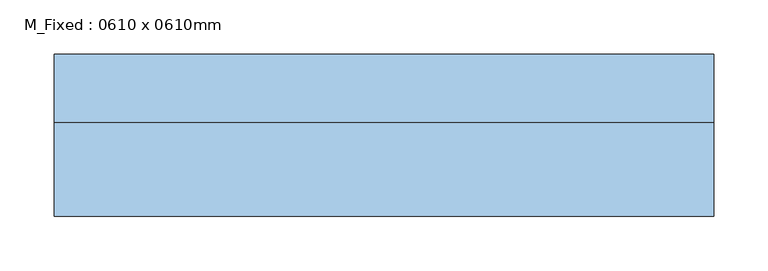
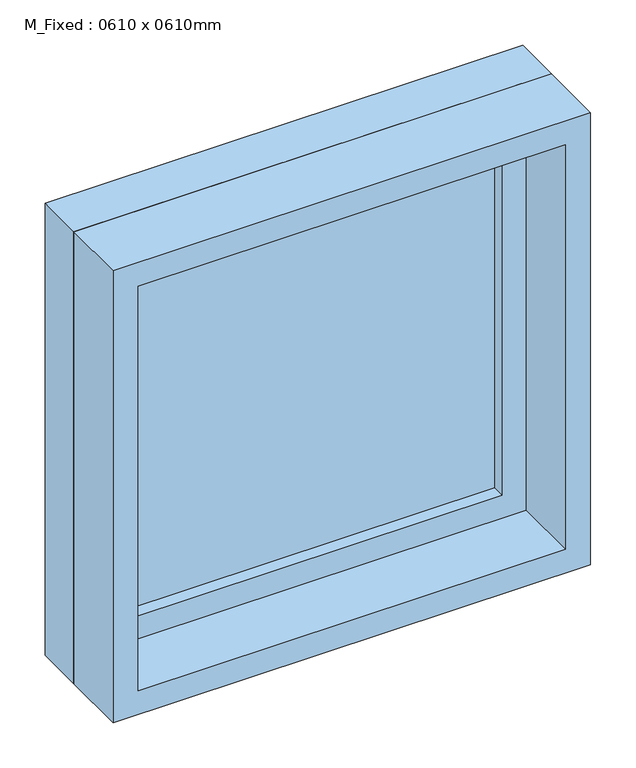
"""IFC4 building model written with IfcOpenShell, lengths in millimetres: window geometry, M_Fixed : 0610 x 0610mm."""

import ifcopenshell
import ifcopenshell.guid

model = None  # the IFC model being written
_history = None  # IfcOwnerHistory: only IFC2X3 demands one
_inside = {}  # id of a spatial element -> (the spatial element, [elements in it])
_under = {}  # id of a project, library or spatial element -> (it, [spatial elements below it])
_declared = {}  # id of a project -> (the project, [libraries it declares])
_typed = {}  # id of a type object -> (the type object, [elements of that type])
_made_of = {}  # id of a material, layer set ... -> (it, [elements and type objects made of it])


def new_model(schema):
    """Start an empty IFC model of exactly this schema.

    Asked for "IFC4X3", IfcOpenShell would pick the latest addendum, in which some entities
    have other attributes; the version numbers below select the first issue.
    IFC2X3 requires an IfcOwnerHistory on every rooted entity: one is made here for all.
    """
    global model, _history
    if schema == "IFC4X3":
        model = ifcopenshell.file(schema_version=(4, 3, 0, 0))
    else:
        model = ifcopenshell.file(schema=schema)
    _inside.clear()
    _under.clear()
    _declared.clear()
    _typed.clear()
    _made_of.clear()
    _history = None
    if model.schema == "IFC2X3":
        org = make("IfcOrganization", Name="unknown")
        user = make(
            "IfcPersonAndOrganization",
            ThePerson=make("IfcPerson", FamilyName="unknown"),
            TheOrganization=org,
        )
        app = make(
            "IfcApplication",
            ApplicationDeveloper=org,
            Version="unknown",
            ApplicationFullName="unknown",
            ApplicationIdentifier="unknown",
        )
        _history = make(
            "IfcOwnerHistory",
            OwningUser=user,
            OwningApplication=app,
            ChangeAction="ADDED",
            CreationDate=0,
        )
    return model


def make(cls, **values):
    """One entity of the class cls with the attributes given. An attribute that is None is left unset."""
    return model.create_entity(
        cls, **{name: value for name, value in values.items() if value is not None}
    )


def rooted(cls, **values):
    """An entity with a GlobalId (a new one), such as an element, a storey or a relation."""
    return make(cls, GlobalId=ifcopenshell.guid.new(), OwnerHistory=_history, **values)


def si_unit(unit_type, name, prefix=None):
    """IfcSIUnit, for example si_unit("LENGTHUNIT", "METRE", prefix="MILLI")."""
    return make("IfcSIUnit", UnitType=unit_type, Prefix=prefix, Name=name)


def assignment(units):
    """IfcUnitAssignment: the units of a project."""
    return None if units is None else make("IfcUnitAssignment", Units=units)


def point(xyz):
    """IfcCartesianPoint."""
    return None if xyz is None else make("IfcCartesianPoint", Coordinates=xyz)


def direction(xyz):
    """IfcDirection."""
    return None if xyz is None else make("IfcDirection", DirectionRatios=xyz)


def frame(location, z_axis=None, x_axis=None):
    """IfcAxis2Placement3D, a coordinate frame: its origin and axes. An axis left out is left unset."""
    return make(
        "IfcAxis2Placement3D",
        Location=point(location),
        Axis=direction(z_axis),
        RefDirection=direction(x_axis),
    )


def origin():
    """The frame at (0, 0, 0) with its axes left unset."""
    return frame((0.0, 0.0, 0.0))


def place(relative_to, where):
    """IfcLocalPlacement: puts the frame where relative to a parent placement (None: the world)."""
    return make(
        "IfcLocalPlacement", PlacementRelTo=relative_to, RelativePlacement=where
    )


def context(
    kind, dimensions, precision=None, world=None, true_north=None, identifier=None
):
    """IfcGeometricRepresentationContext, for example the 3D "Model" context."""
    return make(
        "IfcGeometricRepresentationContext",
        ContextIdentifier=identifier,
        ContextType=kind,
        CoordinateSpaceDimension=dimensions,
        Precision=precision,
        WorldCoordinateSystem=world,
        TrueNorth=true_north,
    )


def project(units=None, contexts=None):
    """IfcProject with its units and contexts."""
    return rooted(
        "IfcProject",
        Name="project",
        RepresentationContexts=contexts,
        UnitsInContext=assignment(units),
    )


def spatial(cls, under=None, at=None, **own):
    """A site, building, storey or space (cls), placed at a placement, below another one or the project."""
    s = rooted(cls, ObjectPlacement=at, **own)
    if under is not None:
        _under.setdefault(under.id(), (under, []))[1].append(s)
    return s


def polyline(points):
    """IfcPolyline through the points."""
    return make("IfcPolyline", Points=[point(p) for p in points])


def outline(outer, holes=None, kind="AREA"):
    """IfcArbitraryClosedProfileDef: a profile drawn as a closed curve; with holes, ...WithVoids."""
    if holes is None:
        return make("IfcArbitraryClosedProfileDef", ProfileType=kind, OuterCurve=outer)
    return make(
        "IfcArbitraryProfileDefWithVoids",
        ProfileType=kind,
        OuterCurve=outer,
        InnerCurves=holes,
    )


def extrude(swept, where, along, depth):
    """IfcExtrudedAreaSolid: the profile swept, set in the frame where, extruded along a direction by depth."""
    return make(
        "IfcExtrudedAreaSolid",
        SweptArea=swept,
        Position=where,
        ExtrudedDirection=direction(along),
        Depth=depth,
    )


def shape(context_of_items, identifier, shape_type, items):
    """IfcShapeRepresentation: the items that make up one representation, for example the "Body"."""
    return make(
        "IfcShapeRepresentation",
        ContextOfItems=context_of_items,
        RepresentationIdentifier=identifier,
        RepresentationType=shape_type,
        Items=items,
    )


def source(mapping_origin, context_of_items, identifier, shape_type, items):
    """IfcRepresentationMap: a shape defined once, which mapped items show again and again."""
    return make(
        "IfcRepresentationMap",
        MappingOrigin=mapping_origin,
        MappedRepresentation=shape(context_of_items, identifier, shape_type, items),
    )


def transform(
    local_origin,
    x_axis=None,
    y_axis=None,
    z_axis=None,
    scale=None,
    scale2=None,
    scale3=None,
    uniform=True,
):
    """IfcCartesianTransformationOperator3D, or its non-uniform kind. x_axis, y_axis, z_axis: its Axis1, 2, 3."""
    if uniform:
        return make(
            "IfcCartesianTransformationOperator3D",
            Axis1=direction(x_axis),
            Axis2=direction(y_axis),
            LocalOrigin=point(local_origin),
            Scale=scale,
            Axis3=direction(z_axis),
        )
    return make(
        "IfcCartesianTransformationOperator3DnonUniform",
        Axis1=direction(x_axis),
        Axis2=direction(y_axis),
        LocalOrigin=point(local_origin),
        Scale=scale,
        Axis3=direction(z_axis),
        Scale2=scale2,
        Scale3=scale3,
    )


def mapped(mapping_source, mapping_target):
    """IfcMappedItem: shows the shape of a source again, moved by a transform."""
    return make(
        "IfcMappedItem", MappingSource=mapping_source, MappingTarget=mapping_target
    )


def made_of(thing, what):
    """Note that an element or type object is made of a material, layer set ...; save() writes the relation."""
    if what is not None:
        _made_of.setdefault(what.id(), (what, []))[1].append(thing)
    return thing


def element(
    cls,
    number,
    at=None,
    inside=None,
    cuts=None,
    type_object=None,
    material=None,
    context=None,
    identifier="Body",
    shape_type=None,
    held_by="IfcProductDefinitionShape",
    body=None,
    shapes=None,
    **own,
):
    """One element of the class cls, such as IfcWall. Its Tag is "e" and its number.

    at: its placement. inside: the storey or other place that contains it. cuts: it is an
    opening in that element (IfcRelVoidsElement). A single representation is given by context,
    identifier, shape_type and body (its items); several are given by shapes. held_by: the class
    of the entity that holds the representations. save() writes the other relations.
    """
    e = rooted(cls, Tag="e%d" % number, ObjectPlacement=at, **own)
    if body is not None:
        shapes = [shape(context, identifier, shape_type, body)]
    if shapes is not None:
        e.Representation = make(held_by, Representations=shapes)
    if inside is not None:
        _inside.setdefault(inside.id(), (inside, []))[1].append(e)
    if cuts is not None:
        rooted(
            "IfcRelVoidsElement", RelatingBuildingElement=cuts, RelatedOpeningElement=e
        )
    if type_object is not None:
        _typed.setdefault(type_object.id(), (type_object, []))[1].append(e)
    return made_of(e, material)


def aggregate(whole, parts):
    """IfcRelAggregates: a whole, such as a stair, and the parts it consists of."""
    return rooted("IfcRelAggregates", RelatingObject=whole, RelatedObjects=parts)


def save(model, path):
    """Write the relations noted so far, then the file.

    IfcRelAggregates (storeys below a building ...), IfcRelContainedInSpatialStructure (elements
    in a storey), IfcRelDefinesByType, IfcRelAssociatesMaterial and IfcRelDeclares: one each for
    every whole, place, type object, material and project.
    """
    for whole, parts in _under.values():
        aggregate(whole, parts)
    for where, things in _inside.values():
        rooted(
            "IfcRelContainedInSpatialStructure",
            RelatedElements=things,
            RelatingStructure=where,
        )
    for kind, things in _typed.values():
        rooted("IfcRelDefinesByType", RelatedObjects=things, RelatingType=kind)
    for what, things in _made_of.values():
        rooted("IfcRelAssociatesMaterial", RelatedObjects=things, RelatingMaterial=what)
    for by, libraries in _declared.values():
        rooted("IfcRelDeclares", RelatingContext=by, RelatedDefinitions=libraries)
    model.write(path)


def m_fixed_0610_x_0610mm_d1ac9692(model_context):
    return source(origin(), model_context, "Body", "SweptSolid", [
        extrude(outline(polyline([(-242.0, 53.0), (242.0, 53.0), (242.0, 41.0), (-242.0, 41.0), (-242.0, 53.0)])), frame((0.0, 0.0, 978.0), z_axis=(0.0, 0.0, 1.0), x_axis=(1.0, 0.0, 0.0)), (0.0, 0.0, 1.0), 484.0),
        extrude(outline(polyline([(1506.0, -286.0), (934.0, -286.0), (934.0, 286.0), (1506.0, 286.0), (1506.0, -286.0)]), holes=[polyline([(1462.0, -242.0), (1462.0, 242.0), (978.0, 242.0), (978.0, -242.0), (1462.0, -242.0)])]), frame((0.0, 25.0, 0.0), z_axis=(0.0, 1.0, 0.0), x_axis=(0.0, 0.0, 1.0)), (0.0, 0.0, 1.0), 44.0),
        extrude(outline(polyline([(1525.0, -305.0), (915.0, -305.0), (915.0, 305.0), (1525.0, 305.0), (1525.0, -305.0)]), holes=[polyline([(1506.0, -286.0), (1506.0, 286.0), (934.0, 286.0), (934.0, -286.0), (1506.0, -286.0)])]), frame((0.0, 25.0, 0.0), z_axis=(0.0, 1.0, 0.0), x_axis=(0.0, 0.0, 1.0)), (0.0, 0.0, 1.0), 63.0),
        extrude(outline(polyline([(1525.0, -305.0), (915.0, -305.0), (915.0, 305.0), (1525.0, 305.0), (1525.0, -305.0)]), holes=[polyline([(1493.0, -273.0), (1493.0, 273.0), (947.0, 273.0), (947.0, -273.0), (1493.0, -273.0)])]), frame((0.0, -62.0, 0.0), z_axis=(0.0, 1.0, 0.0), x_axis=(0.0, 0.0, 1.0)), (0.0, 0.0, 1.0), 87.0),
    ])


if __name__ == "__main__":
    model = new_model("IFC4")
    model_context = context("Model", 3, world=origin())
    ifc_project = project(units=[si_unit("LENGTHUNIT", "METRE", prefix="MILLI")], contexts=[model_context])
    site = spatial("IfcSite", under=ifc_project)
    building = spatial("IfcBuilding", under=site)
    placement = place(None, origin())
    m_fixed_0610_x_0610mm_shape = m_fixed_0610_x_0610mm_d1ac9692(model_context)
    element("IfcWindow", 1, ObjectType="M_Fixed : 0610 x 0610mm", at=placement, inside=building, context=model_context, shape_type="MappedRepresentation", body=[
        mapped(m_fixed_0610_x_0610mm_shape, transform((0.0, 0.0, 0.0), x_axis=(1.0, 0.0, 0.0), y_axis=(0.0, 1.0, 0.0), z_axis=(0.0, 0.0, 1.0))),
    ])
    save(model, "model.ifc")

# Revit data of these elements
# Type "M_Fixed : 0610 x 0610mm"
#   Type Mark = "12"
#   Height = 0.61 m
#   Default Sill Height = 0.915 m
#   Width = 0.61 m
#   Window Inset = 0.019 m
#   Frame Exterior Material = Sash
#   Frame Interior Material = Sash
#   Glass Pane Material = Glass
#   Sash = Sash
#   Wall Closure = (empty or 0)
# Element 1 (IfcWindow, "M_Fixed : 0610 x 0610mm")
#   Materials on its faces: "Sash", "Glass"
# Materials
#   "Sash": class "Wood", colour RGB 136 99 55, transparency 0
#   "Glass": class "Glass", colour RGB 218 227 224, transparency 0.85, Description = "Soda Lime Glass", Cost = 0
